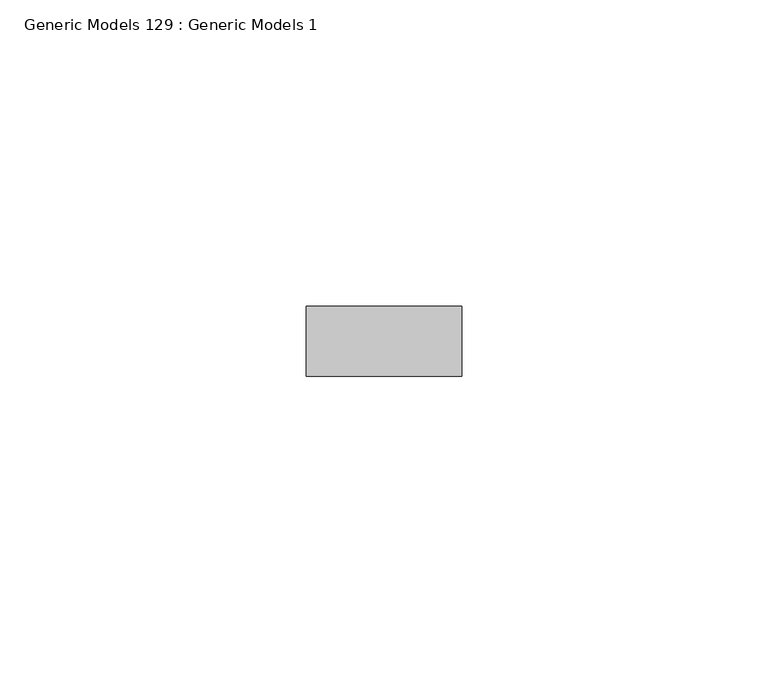
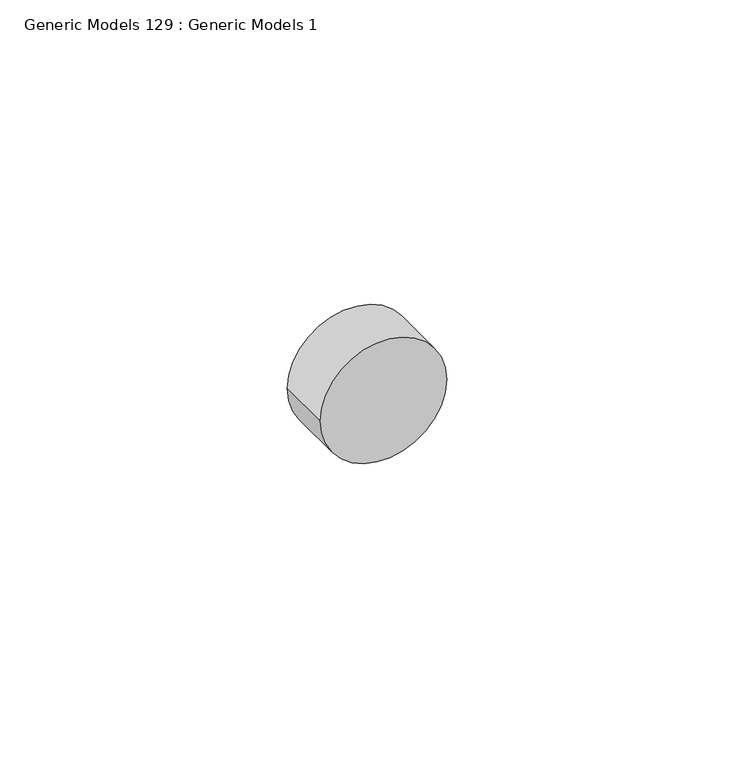
"""IFC4 building model written with IfcOpenShell, lengths in millimetres: proxy geometry, Generic Models 129 : Generic Models 1."""

from ifc_helpers import new_model, si_unit, point, frame, frame_2d, origin, place, context, project, spatial, circle_curve, trimmed, segment, composite_curve, outline, extrude, source, transform, mapped, element, save


def generic_models_129_generic_models_1_ab13da1a(model_context):
    return source(origin(), model_context, "Body", "SweptSolid", [
        extrude(outline(composite_curve([segment(trimmed(circle_curve(frame_2d((38546.4677238, 7966.3828124)), 12.7), [point((38546.4677238, 7953.6828124))], [point((38546.4677238, 7979.0828124))], False, "CARTESIAN"), True, "CONTINUOUS"), segment(trimmed(circle_curve(frame_2d((38546.4677238, 7966.3828124)), 12.7), [point((38546.4677238, 7979.0828124))], [point((38546.4677238, 7953.6828124))], False, "CARTESIAN"), True, "CONTINUOUS")], self_intersect=False)), frame((0.0, 1836.9202358, 0.0), z_axis=(0.0, 1.0, 0.0), x_axis=(0.0, 0.0, 1.0)), (0.0, 0.0, 1.0), 11.4464372),
    ])


if __name__ == "__main__":
    model = new_model("IFC4")
    model_context = context("Model", 3, world=origin())
    ifc_project = project(units=[si_unit("LENGTHUNIT", "METRE", prefix="MILLI")], contexts=[model_context])
    site = spatial("IfcSite", under=ifc_project)
    building = spatial("IfcBuilding", under=site)
    placement = place(None, origin())
    generic_models_129_generic_models_1_shape = generic_models_129_generic_models_1_ab13da1a(model_context)
    element("IfcBuildingElementProxy", 1, Name="Generic Models 129 : Generic Models 1", ObjectType="Generic Models 129 : Generic Models 1", at=placement, inside=building, context=model_context, shape_type="MappedRepresentation", body=[
        mapped(generic_models_129_generic_models_1_shape, transform((0.0, 0.0, 0.0), x_axis=(1.0, 0.0, 0.0), y_axis=(0.0, 1.0, 0.0), z_axis=(0.0, 0.0, 1.0))),
    ])
    save(model, "model.ifc")

# Revit data of these elements
# Element 1 (IfcBuildingElementProxy, "Generic Models 129 : Generic Models 1")
#   Materials on its faces: "S.S. LAG BOLT - SEE STRUCT. DWGS"
# Materials
#   "S.S. LAG BOLT - SEE STRUCT. DWGS": class "Generic", colour RGB 120 120 120, transparency 0, Cost = 0
